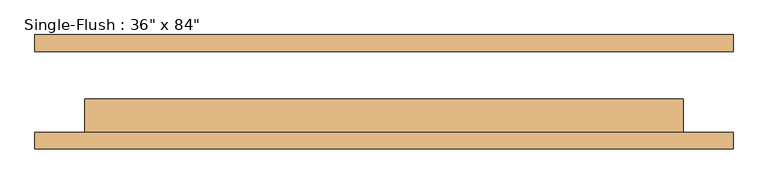
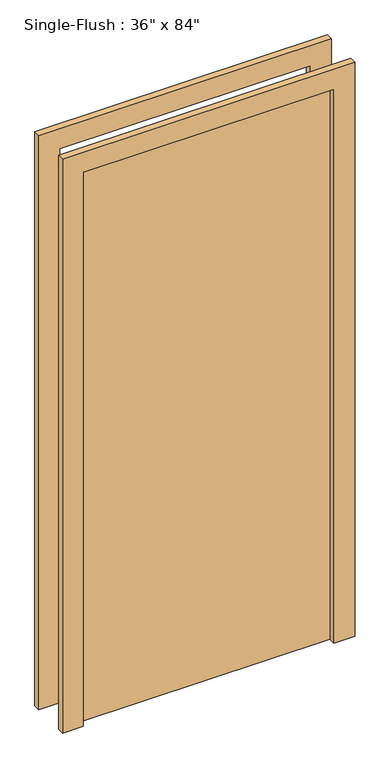
"""IFC4 building model written with IfcOpenShell, lengths in millimetres: door geometry."""

import ifcopenshell
import ifcopenshell.guid

model = None  # the IFC model being written
_history = None  # IfcOwnerHistory: only IFC2X3 demands one
_inside = {}  # id of a spatial element -> (the spatial element, [elements in it])
_under = {}  # id of a project, library or spatial element -> (it, [spatial elements below it])
_declared = {}  # id of a project -> (the project, [libraries it declares])
_typed = {}  # id of a type object -> (the type object, [elements of that type])
_made_of = {}  # id of a material, layer set ... -> (it, [elements and type objects made of it])


def new_model(schema):
    """Start an empty IFC model of exactly this schema.

    Asked for "IFC4X3", IfcOpenShell would pick the latest addendum, in which some entities
    have other attributes; the version numbers below select the first issue.
    IFC2X3 requires an IfcOwnerHistory on every rooted entity: one is made here for all.
    """
    global model, _history
    if schema == "IFC4X3":
        model = ifcopenshell.file(schema_version=(4, 3, 0, 0))
    else:
        model = ifcopenshell.file(schema=schema)
    _inside.clear()
    _under.clear()
    _declared.clear()
    _typed.clear()
    _made_of.clear()
    _history = None
    if model.schema == "IFC2X3":
        org = make("IfcOrganization", Name="unknown")
        user = make(
            "IfcPersonAndOrganization",
            ThePerson=make("IfcPerson", FamilyName="unknown"),
            TheOrganization=org,
        )
        app = make(
            "IfcApplication",
            ApplicationDeveloper=org,
            Version="unknown",
            ApplicationFullName="unknown",
            ApplicationIdentifier="unknown",
        )
        _history = make(
            "IfcOwnerHistory",
            OwningUser=user,
            OwningApplication=app,
            ChangeAction="ADDED",
            CreationDate=0,
        )
    return model


def make(cls, **values):
    """One entity of the class cls with the attributes given. An attribute that is None is left unset."""
    return model.create_entity(
        cls, **{name: value for name, value in values.items() if value is not None}
    )


def rooted(cls, **values):
    """An entity with a GlobalId (a new one), such as an element, a storey or a relation."""
    return make(cls, GlobalId=ifcopenshell.guid.new(), OwnerHistory=_history, **values)


def si_unit(unit_type, name, prefix=None):
    """IfcSIUnit, for example si_unit("LENGTHUNIT", "METRE", prefix="MILLI")."""
    return make("IfcSIUnit", UnitType=unit_type, Prefix=prefix, Name=name)


def assignment(units):
    """IfcUnitAssignment: the units of a project."""
    return None if units is None else make("IfcUnitAssignment", Units=units)


def point(xyz):
    """IfcCartesianPoint."""
    return None if xyz is None else make("IfcCartesianPoint", Coordinates=xyz)


def direction(xyz):
    """IfcDirection."""
    return None if xyz is None else make("IfcDirection", DirectionRatios=xyz)


def frame(location, z_axis=None, x_axis=None):
    """IfcAxis2Placement3D, a coordinate frame: its origin and axes. An axis left out is left unset."""
    return make(
        "IfcAxis2Placement3D",
        Location=point(location),
        Axis=direction(z_axis),
        RefDirection=direction(x_axis),
    )


def origin():
    """The frame at (0, 0, 0) with its axes left unset."""
    return frame((0.0, 0.0, 0.0))


def origin_with_axes():
    """The frame at (0, 0, 0) with the z axis (0, 0, 1) and the x axis (1, 0, 0) written out."""
    return frame((0.0, 0.0, 0.0), z_axis=(0.0, 0.0, 1.0), x_axis=(1.0, 0.0, 0.0))


def place(relative_to, where):
    """IfcLocalPlacement: puts the frame where relative to a parent placement (None: the world)."""
    return make(
        "IfcLocalPlacement", PlacementRelTo=relative_to, RelativePlacement=where
    )


def context(
    kind, dimensions, precision=None, world=None, true_north=None, identifier=None
):
    """IfcGeometricRepresentationContext, for example the 3D "Model" context."""
    return make(
        "IfcGeometricRepresentationContext",
        ContextIdentifier=identifier,
        ContextType=kind,
        CoordinateSpaceDimension=dimensions,
        Precision=precision,
        WorldCoordinateSystem=world,
        TrueNorth=true_north,
    )


def project(units=None, contexts=None):
    """IfcProject with its units and contexts."""
    return rooted(
        "IfcProject",
        Name="project",
        RepresentationContexts=contexts,
        UnitsInContext=assignment(units),
    )


def spatial(cls, under=None, at=None, **own):
    """A site, building, storey or space (cls), placed at a placement, below another one or the project."""
    s = rooted(cls, ObjectPlacement=at, **own)
    if under is not None:
        _under.setdefault(under.id(), (under, []))[1].append(s)
    return s


def polyline(points):
    """IfcPolyline through the points."""
    return make("IfcPolyline", Points=[point(p) for p in points])


def outline(outer, holes=None, kind="AREA"):
    """IfcArbitraryClosedProfileDef: a profile drawn as a closed curve; with holes, ...WithVoids."""
    if holes is None:
        return make("IfcArbitraryClosedProfileDef", ProfileType=kind, OuterCurve=outer)
    return make(
        "IfcArbitraryProfileDefWithVoids",
        ProfileType=kind,
        OuterCurve=outer,
        InnerCurves=holes,
    )


def extrude(swept, where, along, depth):
    """IfcExtrudedAreaSolid: the profile swept, set in the frame where, extruded along a direction by depth."""
    return make(
        "IfcExtrudedAreaSolid",
        SweptArea=swept,
        Position=where,
        ExtrudedDirection=direction(along),
        Depth=depth,
    )


def shape(context_of_items, identifier, shape_type, items):
    """IfcShapeRepresentation: the items that make up one representation, for example the "Body"."""
    return make(
        "IfcShapeRepresentation",
        ContextOfItems=context_of_items,
        RepresentationIdentifier=identifier,
        RepresentationType=shape_type,
        Items=items,
    )


def source(mapping_origin, context_of_items, identifier, shape_type, items):
    """IfcRepresentationMap: a shape defined once, which mapped items show again and again."""
    return make(
        "IfcRepresentationMap",
        MappingOrigin=mapping_origin,
        MappedRepresentation=shape(context_of_items, identifier, shape_type, items),
    )


def transform(
    local_origin,
    x_axis=None,
    y_axis=None,
    z_axis=None,
    scale=None,
    scale2=None,
    scale3=None,
    uniform=True,
):
    """IfcCartesianTransformationOperator3D, or its non-uniform kind. x_axis, y_axis, z_axis: its Axis1, 2, 3."""
    if uniform:
        return make(
            "IfcCartesianTransformationOperator3D",
            Axis1=direction(x_axis),
            Axis2=direction(y_axis),
            LocalOrigin=point(local_origin),
            Scale=scale,
            Axis3=direction(z_axis),
        )
    return make(
        "IfcCartesianTransformationOperator3DnonUniform",
        Axis1=direction(x_axis),
        Axis2=direction(y_axis),
        LocalOrigin=point(local_origin),
        Scale=scale,
        Axis3=direction(z_axis),
        Scale2=scale2,
        Scale3=scale3,
    )


def mapped(mapping_source, mapping_target):
    """IfcMappedItem: shows the shape of a source again, moved by a transform."""
    return make(
        "IfcMappedItem", MappingSource=mapping_source, MappingTarget=mapping_target
    )


def made_of(thing, what):
    """Note that an element or type object is made of a material, layer set ...; save() writes the relation."""
    if what is not None:
        _made_of.setdefault(what.id(), (what, []))[1].append(thing)
    return thing


def element(
    cls,
    number,
    at=None,
    inside=None,
    cuts=None,
    type_object=None,
    material=None,
    context=None,
    identifier="Body",
    shape_type=None,
    held_by="IfcProductDefinitionShape",
    body=None,
    shapes=None,
    **own,
):
    """One element of the class cls, such as IfcWall. Its Tag is "e" and its number.

    at: its placement. inside: the storey or other place that contains it. cuts: it is an
    opening in that element (IfcRelVoidsElement). A single representation is given by context,
    identifier, shape_type and body (its items); several are given by shapes. held_by: the class
    of the entity that holds the representations. save() writes the other relations.
    """
    e = rooted(cls, Tag="e%d" % number, ObjectPlacement=at, **own)
    if body is not None:
        shapes = [shape(context, identifier, shape_type, body)]
    if shapes is not None:
        e.Representation = make(held_by, Representations=shapes)
    if inside is not None:
        _inside.setdefault(inside.id(), (inside, []))[1].append(e)
    if cuts is not None:
        rooted(
            "IfcRelVoidsElement", RelatingBuildingElement=cuts, RelatedOpeningElement=e
        )
    if type_object is not None:
        _typed.setdefault(type_object.id(), (type_object, []))[1].append(e)
    return made_of(e, material)


def aggregate(whole, parts):
    """IfcRelAggregates: a whole, such as a stair, and the parts it consists of."""
    return rooted("IfcRelAggregates", RelatingObject=whole, RelatedObjects=parts)


def save(model, path):
    """Write the relations noted so far, then the file.

    IfcRelAggregates (storeys below a building ...), IfcRelContainedInSpatialStructure (elements
    in a storey), IfcRelDefinesByType, IfcRelAssociatesMaterial and IfcRelDeclares: one each for
    every whole, place, type object, material and project.
    """
    for whole, parts in _under.values():
        aggregate(whole, parts)
    for where, things in _inside.values():
        rooted(
            "IfcRelContainedInSpatialStructure",
            RelatedElements=things,
            RelatingStructure=where,
        )
    for kind, things in _typed.values():
        rooted("IfcRelDefinesByType", RelatedObjects=things, RelatingType=kind)
    for what, things in _made_of.values():
        rooted("IfcRelAssociatesMaterial", RelatedObjects=things, RelatingMaterial=what)
    for by, libraries in _declared.values():
        rooted("IfcRelDeclares", RelatingContext=by, RelatedDefinitions=libraries)
    model.write(path)


def door_eb9f8b14(model_context):
    return source(origin(), model_context, "Body", "SweptSolid", [
        extrude(outline(polyline([(2209.8, -533.4), (0.0, -533.4), (0.0, -457.2), (2133.6, -457.2), (2133.6, 457.2), (0.0, 457.2), (0.0, 533.4), (2209.8, 533.4), (2209.8, -533.4)])), frame((0.0, -87.3125, 0.0), z_axis=(0.0, 1.0, 0.0), x_axis=(0.0, 0.0, 1.0)), (0.0, 0.0, 1.0), 25.4),
        extrude(outline(polyline([(2209.8, 533.4), (2209.8, -533.4), (0.0, -533.4), (0.0, -457.2), (2133.6, -457.2), (2133.6, 457.2), (0.0, 457.2), (0.0, 533.4), (2209.8, 533.4)])), frame((0.0, 61.9125, 0.0), z_axis=(0.0, 1.0, 0.0), x_axis=(0.0, 0.0, 1.0)), (0.0, 0.0, 1.0), 25.4),
        extrude(outline(polyline([(457.2, -11.1125), (457.2, -61.9125), (-457.2, -61.9125), (-457.2, -11.1125), (457.2, -11.1125)])), origin_with_axes(), (0.0, 0.0, 1.0), 2133.6),
    ])


if __name__ == "__main__":
    model = new_model("IFC4")
    model_context = context("Model", 3, world=origin())
    ifc_project = project(units=[si_unit("LENGTHUNIT", "METRE", prefix="MILLI")], contexts=[model_context])
    site = spatial("IfcSite", under=ifc_project)
    building = spatial("IfcBuilding", under=site)
    placement = place(None, origin())
    door_shape = door_eb9f8b14(model_context)
    element("IfcDoor", 1, ObjectType="Single-Flush : 36\" x 84\"", at=placement, inside=building, context=model_context, shape_type="MappedRepresentation", body=[
        mapped(door_shape, transform((0.0, 0.0, 0.0), x_axis=(1.0, 0.0, 0.0), y_axis=(0.0, 1.0, 0.0), z_axis=(0.0, 0.0, 1.0))),
    ])
    save(model, "model.ifc")

# Revit data of these elements
# Type "Single-Flush : 36\" x 84\""
#   Type Mark = "1"
#   Construction Type = "A"
#   Construction Type = "A"
#   Assembly Code = "C1020"
#   Thickness = 0' - 2"
#   Height = 7' - 0"
#   Trim Projection Ext = 0' - 1"
#   Trim Projection Int = 0' - 1"
#   Trim Width = 0' - 3"
#   Width = 3' - 0"
#   Door Material = Door - Panel
#   Frame Material = Door - Frame
#   Function = (empty or 0)
#   Wall Closure = (empty or 0)
# Element 1 (IfcDoor, "Single-Flush : 36\" x 84\"")
#   Materials on its faces: "Door - Frame", "Door - Panel"
# Materials
#   "Door - Panel": class "Wood", colour RGB 210 159 95, transparency 0
#   "Door - Frame": class "Miscellaneous", colour RGB 118 70 51, transparency 0
